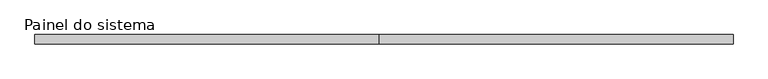
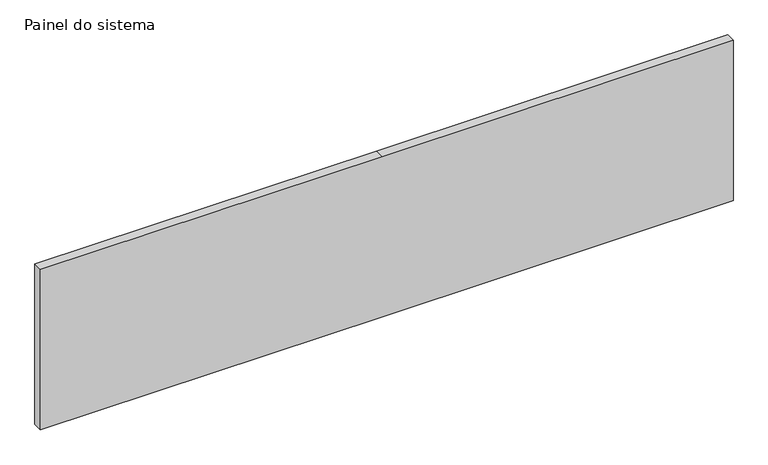
"""IFC4 building model written with IfcOpenShell, lengths in millimetres: plate geometry, Painel do sistema : Envidraçado."""

from ifc_helpers import new_model, si_unit, frame, origin, place, context, project, spatial, polyline, outline, extrude, source, transform, mapped, element, save


def painel_do_sistema_ef095440(model_context):
    return source(origin(), model_context, "Body", "SweptSolid", [
        extrude(outline(polyline([(0.0, -918.5166667), (0.0, -12.4999998), (0.0, 918.5166667), (450.0, 918.5166667), (450.0, -12.4999998), (450.0, -918.5166667), (0.0, -918.5166667)])), frame((0.0, 24.5, 0.0), z_axis=(0.0, 1.0, 0.0), x_axis=(0.0, 0.0, 1.0)), (0.0, 0.0, 1.0), 25.0),
    ])


if __name__ == "__main__":
    model = new_model("IFC4")
    model_context = context("Model", 3, world=origin())
    ifc_project = project(units=[si_unit("LENGTHUNIT", "METRE", prefix="MILLI")], contexts=[model_context])
    site = spatial("IfcSite", under=ifc_project)
    building = spatial("IfcBuilding", under=site)
    placement = place(None, origin())
    painel_do_sistema_shape = painel_do_sistema_ef095440(model_context)
    element("IfcPlate", 1, ObjectType="Painel do sistema : Envidraçado", at=placement, inside=building, context=model_context, shape_type="MappedRepresentation", body=[
        mapped(painel_do_sistema_shape, transform((0.0, 0.0, 0.0), x_axis=(1.0, 0.0, 0.0), y_axis=(0.0, 1.0, 0.0), z_axis=(0.0, 0.0, 1.0))),
    ])
    save(model, "model.ifc")

# Revit data of these elements
# Type "Painel do sistema : Envidraçado"
#   Construction Type Id = "GSP4R"
#   Analytic Construction = "Vidraça única Pilkington 1/8 pol"
#   Visual Light Transmittance = 0.9
#   Solar Heat Gain Coefficient = 0.86
#   Heat Transfer Coefficient (U) = 6.7069 W/(m²·K)
# Element 1 (IfcPlate, "Painel do sistema : Envidraçado")
#   Materials on its faces: ".VIDRO GENÉRICO"
# Materials
#   ".VIDRO GENÉRICO": class ".CC_VIDRO", colour RGB 0 128 192, transparency 0.9, Description = "Vidro comum", Cost = 0
